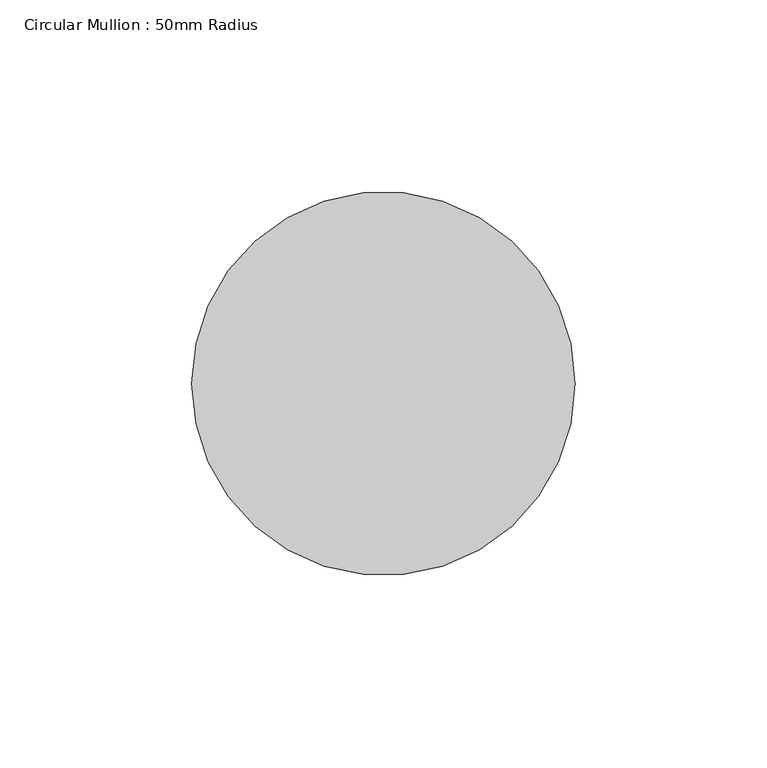
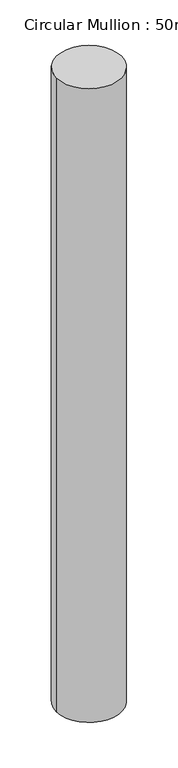
"""IFC4 building model written with IfcOpenShell, lengths in millimetres: member geometry, Circular Mullion : 50mm Radius."""

from ifc_helpers import new_model, si_unit, point, frame, origin, origin_2d, place, context, project, spatial, circle_curve, trimmed, segment, composite_curve, outline, extrude, source, transform, mapped, element, save


def circular_mullion_50mm_radius_85692127(model_context):
    return source(origin(), model_context, "Body", "SweptSolid", [
        extrude(outline(composite_curve([segment(trimmed(circle_curve(origin_2d(), 50.0), [point((50.0, 0.0))], [point((-50.0, 0.0))], False, "CARTESIAN"), True, "CONTINUOUS"), segment(trimmed(circle_curve(origin_2d(), 50.0), [point((-50.0, 0.0))], [point((50.0, 0.0))], False, "CARTESIAN"), True, "CONTINUOUS")], self_intersect=False)), frame((0.0, 0.0, -1028.9879046), z_axis=(0.0, 0.0, 1.0), x_axis=(1.0, 0.0, 0.0)), (0.0, 0.0, 1.0), 1028.9879046),
    ])


if __name__ == "__main__":
    model = new_model("IFC4")
    model_context = context("Model", 3, world=origin())
    ifc_project = project(units=[si_unit("LENGTHUNIT", "METRE", prefix="MILLI")], contexts=[model_context])
    site = spatial("IfcSite", under=ifc_project)
    building = spatial("IfcBuilding", under=site)
    placement = place(None, origin())
    circular_mullion_50mm_radius_shape = circular_mullion_50mm_radius_85692127(model_context)
    element("IfcMember", 1, ObjectType="Circular Mullion : 50mm Radius", at=placement, inside=building, context=model_context, shape_type="MappedRepresentation", body=[
        mapped(circular_mullion_50mm_radius_shape, transform((0.0, 0.0, 0.0), x_axis=(1.0, 0.0, 0.0), y_axis=(0.0, 1.0, 0.0), z_axis=(0.0, 0.0, 1.0))),
    ])
    save(model, "model.ifc")

# Revit data of these elements
# Type "Circular Mullion : 50mm Radius"
#   built-in parameter 1007350 = 0.164042 (stored number, unit not read)
# Element 1 (IfcMember, "Circular Mullion : 50mm Radius")
#   Materials on its faces: "Aluminium"
# Materials
#   "Aluminium": class "Metal", colour RGB 247 247 247, transparency 0, Description = "Aluminium 6061", Cost = 0
